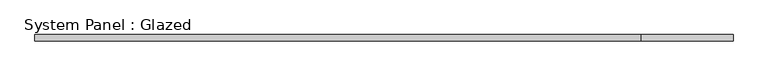
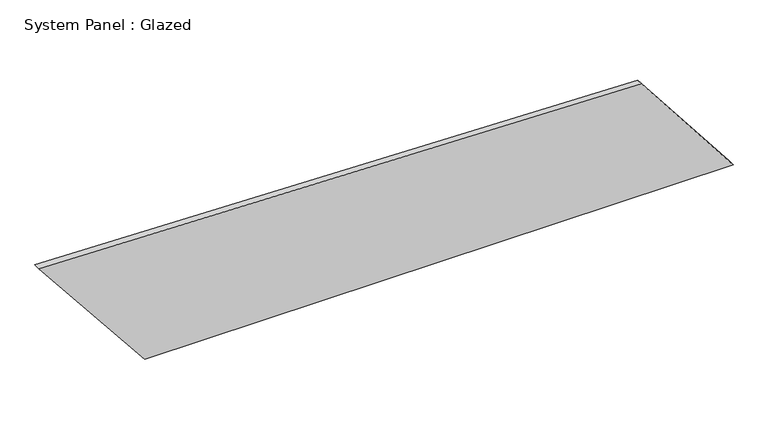
"""IFC4 building model written with IfcOpenShell, lengths in millimetres: plate geometry, System Panel : Glazed."""

import ifcopenshell
import ifcopenshell.guid

model = None  # the IFC model being written
_history = None  # IfcOwnerHistory: only IFC2X3 demands one
_inside = {}  # id of a spatial element -> (the spatial element, [elements in it])
_under = {}  # id of a project, library or spatial element -> (it, [spatial elements below it])
_declared = {}  # id of a project -> (the project, [libraries it declares])
_typed = {}  # id of a type object -> (the type object, [elements of that type])
_made_of = {}  # id of a material, layer set ... -> (it, [elements and type objects made of it])


def new_model(schema):
    """Start an empty IFC model of exactly this schema.

    Asked for "IFC4X3", IfcOpenShell would pick the latest addendum, in which some entities
    have other attributes; the version numbers below select the first issue.
    IFC2X3 requires an IfcOwnerHistory on every rooted entity: one is made here for all.
    """
    global model, _history
    if schema == "IFC4X3":
        model = ifcopenshell.file(schema_version=(4, 3, 0, 0))
    else:
        model = ifcopenshell.file(schema=schema)
    _inside.clear()
    _under.clear()
    _declared.clear()
    _typed.clear()
    _made_of.clear()
    _history = None
    if model.schema == "IFC2X3":
        org = make("IfcOrganization", Name="unknown")
        user = make(
            "IfcPersonAndOrganization",
            ThePerson=make("IfcPerson", FamilyName="unknown"),
            TheOrganization=org,
        )
        app = make(
            "IfcApplication",
            ApplicationDeveloper=org,
            Version="unknown",
            ApplicationFullName="unknown",
            ApplicationIdentifier="unknown",
        )
        _history = make(
            "IfcOwnerHistory",
            OwningUser=user,
            OwningApplication=app,
            ChangeAction="ADDED",
            CreationDate=0,
        )
    return model


def make(cls, **values):
    """One entity of the class cls with the attributes given. An attribute that is None is left unset."""
    return model.create_entity(
        cls, **{name: value for name, value in values.items() if value is not None}
    )


def rooted(cls, **values):
    """An entity with a GlobalId (a new one), such as an element, a storey or a relation."""
    return make(cls, GlobalId=ifcopenshell.guid.new(), OwnerHistory=_history, **values)


def si_unit(unit_type, name, prefix=None):
    """IfcSIUnit, for example si_unit("LENGTHUNIT", "METRE", prefix="MILLI")."""
    return make("IfcSIUnit", UnitType=unit_type, Prefix=prefix, Name=name)


def assignment(units):
    """IfcUnitAssignment: the units of a project."""
    return None if units is None else make("IfcUnitAssignment", Units=units)


def point(xyz):
    """IfcCartesianPoint."""
    return None if xyz is None else make("IfcCartesianPoint", Coordinates=xyz)


def direction(xyz):
    """IfcDirection."""
    return None if xyz is None else make("IfcDirection", DirectionRatios=xyz)


def frame(location, z_axis=None, x_axis=None):
    """IfcAxis2Placement3D, a coordinate frame: its origin and axes. An axis left out is left unset."""
    return make(
        "IfcAxis2Placement3D",
        Location=point(location),
        Axis=direction(z_axis),
        RefDirection=direction(x_axis),
    )


def origin():
    """The frame at (0, 0, 0) with its axes left unset."""
    return frame((0.0, 0.0, 0.0))


def place(relative_to, where):
    """IfcLocalPlacement: puts the frame where relative to a parent placement (None: the world)."""
    return make(
        "IfcLocalPlacement", PlacementRelTo=relative_to, RelativePlacement=where
    )


def context(
    kind, dimensions, precision=None, world=None, true_north=None, identifier=None
):
    """IfcGeometricRepresentationContext, for example the 3D "Model" context."""
    return make(
        "IfcGeometricRepresentationContext",
        ContextIdentifier=identifier,
        ContextType=kind,
        CoordinateSpaceDimension=dimensions,
        Precision=precision,
        WorldCoordinateSystem=world,
        TrueNorth=true_north,
    )


def project(units=None, contexts=None):
    """IfcProject with its units and contexts."""
    return rooted(
        "IfcProject",
        Name="project",
        RepresentationContexts=contexts,
        UnitsInContext=assignment(units),
    )


def spatial(cls, under=None, at=None, **own):
    """A site, building, storey or space (cls), placed at a placement, below another one or the project."""
    s = rooted(cls, ObjectPlacement=at, **own)
    if under is not None:
        _under.setdefault(under.id(), (under, []))[1].append(s)
    return s


def polyline(points):
    """IfcPolyline through the points."""
    return make("IfcPolyline", Points=[point(p) for p in points])


def outline(outer, holes=None, kind="AREA"):
    """IfcArbitraryClosedProfileDef: a profile drawn as a closed curve; with holes, ...WithVoids."""
    if holes is None:
        return make("IfcArbitraryClosedProfileDef", ProfileType=kind, OuterCurve=outer)
    return make(
        "IfcArbitraryProfileDefWithVoids",
        ProfileType=kind,
        OuterCurve=outer,
        InnerCurves=holes,
    )


def extrude(swept, where, along, depth):
    """IfcExtrudedAreaSolid: the profile swept, set in the frame where, extruded along a direction by depth."""
    return make(
        "IfcExtrudedAreaSolid",
        SweptArea=swept,
        Position=where,
        ExtrudedDirection=direction(along),
        Depth=depth,
    )


def shape(context_of_items, identifier, shape_type, items):
    """IfcShapeRepresentation: the items that make up one representation, for example the "Body"."""
    return make(
        "IfcShapeRepresentation",
        ContextOfItems=context_of_items,
        RepresentationIdentifier=identifier,
        RepresentationType=shape_type,
        Items=items,
    )


def source(mapping_origin, context_of_items, identifier, shape_type, items):
    """IfcRepresentationMap: a shape defined once, which mapped items show again and again."""
    return make(
        "IfcRepresentationMap",
        MappingOrigin=mapping_origin,
        MappedRepresentation=shape(context_of_items, identifier, shape_type, items),
    )


def transform(
    local_origin,
    x_axis=None,
    y_axis=None,
    z_axis=None,
    scale=None,
    scale2=None,
    scale3=None,
    uniform=True,
):
    """IfcCartesianTransformationOperator3D, or its non-uniform kind. x_axis, y_axis, z_axis: its Axis1, 2, 3."""
    if uniform:
        return make(
            "IfcCartesianTransformationOperator3D",
            Axis1=direction(x_axis),
            Axis2=direction(y_axis),
            LocalOrigin=point(local_origin),
            Scale=scale,
            Axis3=direction(z_axis),
        )
    return make(
        "IfcCartesianTransformationOperator3DnonUniform",
        Axis1=direction(x_axis),
        Axis2=direction(y_axis),
        LocalOrigin=point(local_origin),
        Scale=scale,
        Axis3=direction(z_axis),
        Scale2=scale2,
        Scale3=scale3,
    )


def mapped(mapping_source, mapping_target):
    """IfcMappedItem: shows the shape of a source again, moved by a transform."""
    return make(
        "IfcMappedItem", MappingSource=mapping_source, MappingTarget=mapping_target
    )


def made_of(thing, what):
    """Note that an element or type object is made of a material, layer set ...; save() writes the relation."""
    if what is not None:
        _made_of.setdefault(what.id(), (what, []))[1].append(thing)
    return thing


def element(
    cls,
    number,
    at=None,
    inside=None,
    cuts=None,
    type_object=None,
    material=None,
    context=None,
    identifier="Body",
    shape_type=None,
    held_by="IfcProductDefinitionShape",
    body=None,
    shapes=None,
    **own,
):
    """One element of the class cls, such as IfcWall. Its Tag is "e" and its number.

    at: its placement. inside: the storey or other place that contains it. cuts: it is an
    opening in that element (IfcRelVoidsElement). A single representation is given by context,
    identifier, shape_type and body (its items); several are given by shapes. held_by: the class
    of the entity that holds the representations. save() writes the other relations.
    """
    e = rooted(cls, Tag="e%d" % number, ObjectPlacement=at, **own)
    if body is not None:
        shapes = [shape(context, identifier, shape_type, body)]
    if shapes is not None:
        e.Representation = make(held_by, Representations=shapes)
    if inside is not None:
        _inside.setdefault(inside.id(), (inside, []))[1].append(e)
    if cuts is not None:
        rooted(
            "IfcRelVoidsElement", RelatingBuildingElement=cuts, RelatedOpeningElement=e
        )
    if type_object is not None:
        _typed.setdefault(type_object.id(), (type_object, []))[1].append(e)
    return made_of(e, material)


def aggregate(whole, parts):
    """IfcRelAggregates: a whole, such as a stair, and the parts it consists of."""
    return rooted("IfcRelAggregates", RelatingObject=whole, RelatedObjects=parts)


def save(model, path):
    """Write the relations noted so far, then the file.

    IfcRelAggregates (storeys below a building ...), IfcRelContainedInSpatialStructure (elements
    in a storey), IfcRelDefinesByType, IfcRelAssociatesMaterial and IfcRelDeclares: one each for
    every whole, place, type object, material and project.
    """
    for whole, parts in _under.values():
        aggregate(whole, parts)
    for where, things in _inside.values():
        rooted(
            "IfcRelContainedInSpatialStructure",
            RelatedElements=things,
            RelatingStructure=where,
        )
    for kind, things in _typed.values():
        rooted("IfcRelDefinesByType", RelatedObjects=things, RelatingType=kind)
    for what, things in _made_of.values():
        rooted("IfcRelAssociatesMaterial", RelatedObjects=things, RelatingMaterial=what)
    for by, libraries in _declared.values():
        rooted("IfcRelDeclares", RelatingContext=by, RelatedDefinitions=libraries)
    model.write(path)


def system_panel_glazed_1eb3be1f(model_context):
    return source(origin(), model_context, "Body", "SweptSolid", [
        extrude(outline(polyline([(0.0, -925.0562456), (0.0, 1333.2930861), (450.8755281, 982.3228685), (511.5308744, -1333.2930861), (0.0, -925.0562456)])), frame((0.0, -49.5, 0.0), z_axis=(0.0, 1.0, 0.0), x_axis=(0.0, 0.0, 1.0)), (0.0, 0.0, 1.0), 25.0),
    ])


if __name__ == "__main__":
    model = new_model("IFC4")
    model_context = context("Model", 3, world=origin())
    ifc_project = project(units=[si_unit("LENGTHUNIT", "METRE", prefix="MILLI")], contexts=[model_context])
    site = spatial("IfcSite", under=ifc_project)
    building = spatial("IfcBuilding", under=site)
    placement = place(None, origin())
    system_panel_glazed_shape = system_panel_glazed_1eb3be1f(model_context)
    element("IfcPlate", 1, ObjectType="System Panel : Glazed", at=placement, inside=building, context=model_context, shape_type="MappedRepresentation", body=[
        mapped(system_panel_glazed_shape, transform((0.0, 0.0, 0.0), x_axis=(1.0, 0.0, 0.0), y_axis=(0.0, 1.0, 0.0), z_axis=(0.0, 0.0, 1.0))),
    ])
    save(model, "model.ifc")

# Revit data of these elements
# Element 1 (IfcPlate, "System Panel : Glazed")
#   Materials on its faces: "Glass, Clear Glazing"
# Materials
#   "Glass, Clear Glazing": class "Glass", colour RGB 247 249 248, transparency 0.85, Description = "Clear glazing", Cost = 0
